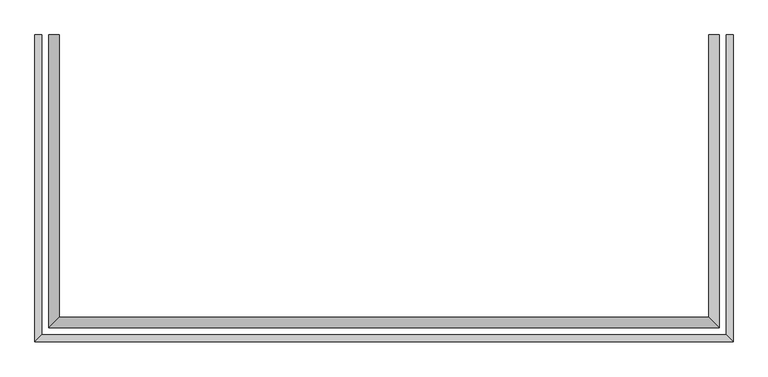
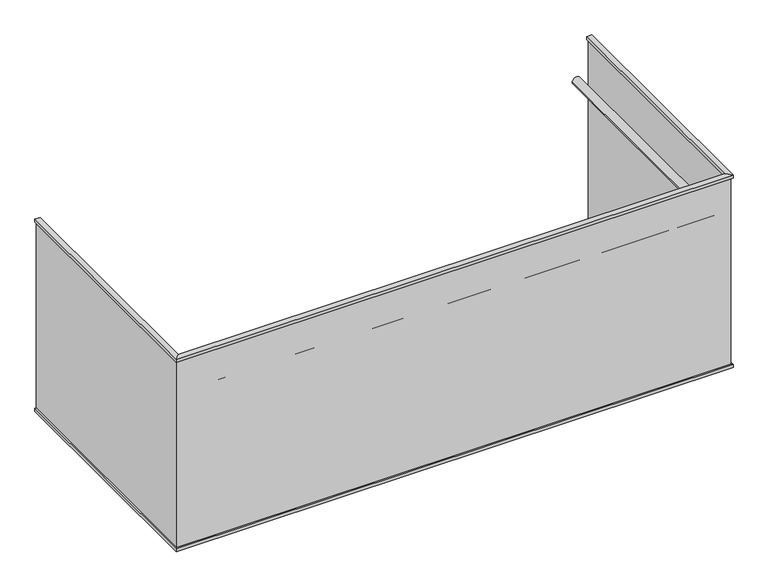
"""IFC4 building model written with IfcOpenShell, lengths in millimetres: railing geometry."""

from ifc_helpers import new_model, si_unit, frame, origin, place, context, project, spatial, circle_curve, ellipse_curve, faceted_brep, source, transform, mapped, element, save
from ifc_brep_helpers import plane_surface, cylinder_surface, advanced_brep


def railing_0fda917e(model_context):
    return source(origin(), model_context, "Body", "SolidModel", [
        faceted_brep([(-54221.6601064, 44661.421627, 1035.0), (-54221.6601064, 44661.421627, 1050.0), (-51631.6653864, 44661.421627, 1050.0), (-51631.6653864, 44661.421627, 1035.0), (-54246.6601064, 44636.421627, 1035.0), (-51606.6653864, 44636.421627, 1035.0), (-54246.6601064, 44636.421627, 1050.0), (-51606.6653864, 44636.421627, 1050.0), (-54221.6601064, 45795.9212804, 1050.0), (-54221.6601064, 45795.9212804, 1035.0), (-54246.6601064, 45795.9212804, 1035.0), (-54246.6601064, 45795.9212804, 1050.0), (-51631.6653864, 45795.9212804, 1050.0), (-51606.6653864, 45795.9212804, 1050.0), (-51606.6653864, 45795.9212804, 1035.0), (-51631.6653864, 45795.9212804, 1035.0)], [[[0, 1, 2, 3]], [[4, 0, 3, 5]], [[6, 4, 5, 7]], [[1, 6, 7, 2]], [[8, 9, 10, 11]], [[8, 11, 6, 1]], [[11, 10, 4, 6]], [[10, 9, 0, 4]], [[9, 8, 1, 0]], [[12, 13, 14, 15]], [[3, 2, 12, 15]], [[5, 3, 15, 14]], [[7, 5, 14, 13]], [[2, 7, 13, 12]]]),
        faceted_brep([(-54229.1601064, 44653.921627, 1040.0), (-54239.1601064, 44643.921627, 1040.0), (-51614.1653864, 44643.921627, 1040.0), (-51624.1653864, 44653.921627, 1040.0), (-54229.1601064, 44653.921627, 90.0), (-51624.1653864, 44653.921627, 90.0), (-54239.1601064, 44643.921627, 90.0), (-51614.1653864, 44643.921627, 90.0), (-54239.1601064, 45795.9212804, 1040.0), (-54229.1601064, 45795.9212804, 1040.0), (-54229.1601064, 45795.9212804, 90.0), (-54239.1601064, 45795.9212804, 90.0), (-51614.1653864, 45795.9212804, 1040.0), (-51614.1653864, 45795.9212804, 90.0), (-51624.1653864, 45795.9212804, 90.0), (-51624.1653864, 45795.9212804, 1040.0)], [[[0, 1, 2, 3]], [[4, 0, 3, 5]], [[6, 4, 5, 7]], [[1, 6, 7, 2]], [[8, 9, 10, 11]], [[8, 11, 6, 1]], [[11, 10, 4, 6]], [[10, 9, 0, 4]], [[9, 8, 1, 0]], [[12, 13, 14, 15]], [[3, 2, 12, 15]], [[5, 3, 15, 14]], [[7, 5, 14, 13]], [[2, 7, 13, 12]]]),
        advanced_brep(
        [(-54194.1601064, 44688.921627, 845.0), (-54154.1601064, 44728.921627, 845.0), (-51699.1653864, 44728.921627, 845.0), (-51659.1653864, 44688.921627, 845.0), (-54154.1601064, 45795.9212804, 845.0), (-54194.1601064, 45795.9212804, 845.0), (-51699.1653864, 45795.9212804, 845.0), (-51659.1653864, 45795.9212804, 845.0)],
        [
            (0, 1, ellipse_curve(frame((-54174.1601064, 44708.921627, 845.0), z_axis=(0.7071067811865391, -0.7071067811865558, 0.0), x_axis=(-0.7071067811865559, -0.7071067811865391, 0.0)), 28.2842712, 20.0)),
            (1, 2),
            (2, 3, ellipse_curve(frame((-51679.1653864, 44708.921627, 845.0), z_axis=(-0.7071067811865479, -0.7071067811865471, 0.0), x_axis=(-0.7071067811865471, 0.7071067811865478, 0.0)), 28.2842712, 20.0)),
            (3, 0),
            (1, 0, ellipse_curve(frame((-54174.1601064, 44708.921627, 845.0), z_axis=(0.7071067811865391, -0.7071067811865558, 0.0), x_axis=(-0.7071067811865559, -0.7071067811865391, 0.0)), 28.2842712, 20.0)),
            (3, 2, ellipse_curve(frame((-51679.1653864, 44708.921627, 845.0), z_axis=(-0.7071067811865479, -0.7071067811865471, 0.0), x_axis=(-0.7071067811865471, 0.7071067811865478, 0.0)), 28.2842712, 20.0)),
            (4, 5, circle_curve(frame((-54174.1601064, 45795.9212804, 845.0), z_axis=(0.0, 1.0, 0.0), x_axis=(-1.0, 0.0, 0.0)), 20.0)),
            (5, 4, circle_curve(frame((-54174.1601064, 45795.9212804, 845.0), z_axis=(0.0, 1.0, 0.0), x_axis=(-1.0, 0.0, 0.0)), 20.0)),
            (5, 0),
            (1, 4),
            (6, 7, circle_curve(frame((-51679.1653864, 45795.9212804, 845.0), z_axis=(0.0, 1.0, 0.0), x_axis=(1.0, 0.0, 0.0)), 20.0)),
            (7, 6, circle_curve(frame((-51679.1653864, 45795.9212804, 845.0), z_axis=(0.0, 1.0, 0.0), x_axis=(1.0, 0.0, 0.0)), 20.0)),
            (2, 6),
            (7, 3),
        ],
        [
            cylinder_surface(frame((-54174.1601064, 44708.921627, 845.0), z_axis=(-1.0, 0.0, 0.0), x_axis=(0.0, -1.0, 0.0)), 20.0),
            plane_surface(frame((-54174.1601064, 45795.9212804, 865.0), z_axis=(0.0, 1.0, 0.0), x_axis=(0.0, 0.0, -1.0))),
            cylinder_surface(frame((-54174.1601064, 45795.9212804, 845.0), z_axis=(0.0, 1.0, 0.0), x_axis=(-1.0, 0.0, 0.0)), 20.0),
            plane_surface(frame((-51679.1653864, 45795.9212804, 865.0), z_axis=(0.0, 1.0, 0.0), x_axis=(0.0, 0.0, 1.0))),
            cylinder_surface(frame((-51679.1653864, 44708.921627, 845.0), z_axis=(0.0, -1.0, 0.0), x_axis=(1.0, 0.0, 0.0)), 20.0),
        ],
        [
            (0, [[1, 2, 3, 4]]),
            (0, [[5, -4, 6, -2]]),
            (1, [[7, 8]]),
            (2, [[-8, 9, -5, 10]]),
            (2, [[-7, -10, -1, -9]]),
            (3, [[11, 12]]),
            (4, [[-3, 13, -12, 14]]),
            (4, [[-6, -14, -11, -13]]),
        ],
    ),
        faceted_brep([(-54221.6601064, 44661.421627, 85.0), (-54221.6601064, 44661.421627, 100.0), (-51631.6653864, 44661.421627, 100.0), (-51631.6653864, 44661.421627, 85.0), (-54246.6601064, 44636.421627, 85.0), (-51606.6653864, 44636.421627, 85.0), (-54246.6601064, 44636.421627, 100.0), (-51606.6653864, 44636.421627, 100.0), (-54221.6601064, 45795.9212804, 100.0), (-54221.6601064, 45795.9212804, 85.0), (-54246.6601064, 45795.9212804, 85.0), (-54246.6601064, 45795.9212804, 100.0), (-51631.6653864, 45795.9212804, 100.0), (-51606.6653864, 45795.9212804, 100.0), (-51606.6653864, 45795.9212804, 85.0), (-51631.6653864, 45795.9212804, 85.0)], [[[0, 1, 2, 3]], [[4, 0, 3, 5]], [[6, 4, 5, 7]], [[1, 6, 7, 2]], [[8, 9, 10, 11]], [[8, 11, 6, 1]], [[11, 10, 4, 6]], [[10, 9, 0, 4]], [[9, 8, 1, 0]], [[12, 13, 14, 15]], [[3, 2, 12, 15]], [[5, 3, 15, 14]], [[7, 5, 14, 13]], [[2, 7, 13, 12]]]),
    ])


if __name__ == "__main__":
    model = new_model("IFC4")
    model_context = context("Model", 3, world=origin())
    ifc_project = project(units=[si_unit("LENGTHUNIT", "METRE", prefix="MILLI")], contexts=[model_context])
    site = spatial("IfcSite", under=ifc_project)
    building = spatial("IfcBuilding", under=site)
    placement = place(None, origin())
    railing_shape = railing_0fda917e(model_context)
    element("IfcRailing", 1, at=placement, inside=building, context=model_context, shape_type="MappedRepresentation", body=[
        mapped(railing_shape, transform((0.0, 0.0, 0.0), x_axis=(1.0, 0.0, 0.0), y_axis=(0.0, 1.0, 0.0), z_axis=(0.0, 0.0, 1.0))),
    ])
    save(model, "model.ifc")

# Revit data of these elements
# Element 1 (IfcRailing)
#   Materials on its faces: "Tempered Glass2", "Stainless Steel2"
# Materials
#   "Tempered Glass2": class "Unassigned", colour RGB 145 219 255, transparency 0.75, Description = "Glass", Cost = 0
#   "Stainless Steel2": class "Metal", colour RGB 203 203 203, transparency 0, Cost = 0
